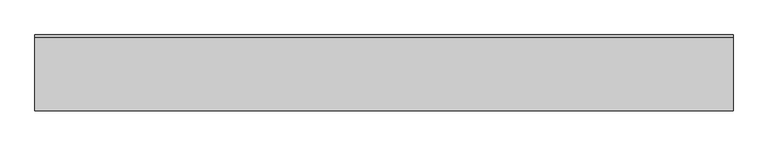
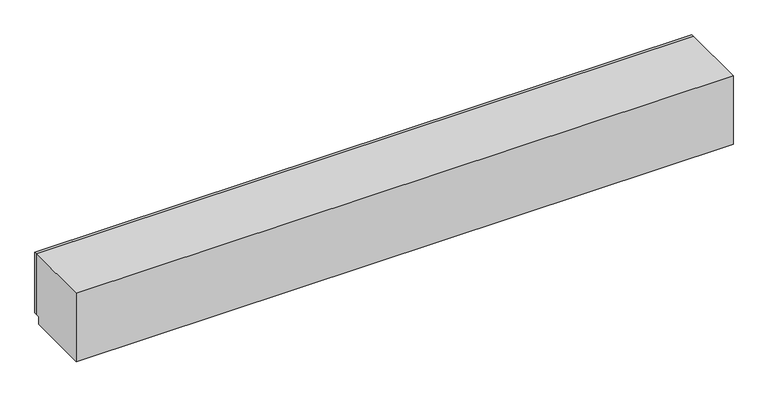
"""IFC4 building model written with IfcOpenShell, lengths in millimetres: furniture geometry, OD_CW_Base Cabinet : OD_CW_Base Cabinet."""

from ifc_helpers import new_model, si_unit, frame, origin, place, context, project, spatial, polyline, outline, extrude, source, transform, mapped, element, save


def furniture_861fb723(model_context):
    return source(origin(), model_context, "Body", "SweptSolid", [
        extrude(outline(polyline([(18.7377049, 228.6), (18.7377049, 254.0), (7982.4770576, 254.0), (7982.4770576, 228.6), (18.7377049, 228.6)])), frame((0.0, 0.0, 101.6), z_axis=(0.0, 0.0, 1.0), x_axis=(1.0, 0.0, 0.0)), (0.0, 0.0, 1.0), 774.7),
        extrude(outline(polyline([(228.6, 876.3), (228.6, 101.6), (177.8, 101.6), (177.8, 0.0), (-609.6, 0.0), (-609.6, 876.3), (228.6, 876.3)])), frame((18.7377049, 0.0, 0.0), z_axis=(1.0, 0.0, 0.0), x_axis=(0.0, 1.0, 0.0)), (0.0, 0.0, 1.0), 7963.7393527),
    ])


if __name__ == "__main__":
    model = new_model("IFC4")
    model_context = context("Model", 3, world=origin())
    ifc_project = project(units=[si_unit("LENGTHUNIT", "METRE", prefix="MILLI")], contexts=[model_context])
    site = spatial("IfcSite", under=ifc_project)
    building = spatial("IfcBuilding", under=site)
    placement = place(None, origin())
    furniture_shape = furniture_861fb723(model_context)
    element("IfcFurniture", 1, ObjectType="OD_CW_Base Cabinet : OD_CW_Base Cabinet", at=placement, inside=building, context=model_context, shape_type="MappedRepresentation", body=[
        mapped(furniture_shape, transform((0.0, 0.0, 0.0), x_axis=(1.0, 0.0, 0.0), y_axis=(0.0, 1.0, 0.0), z_axis=(0.0, 0.0, 1.0))),
    ])
    save(model, "model.ifc")

# Revit data of these elements
# Type "OD_CW_Base Cabinet : OD_CW_Base Cabinet"
#   OD_CW_Width [instance default] = 2' - 10"
#   OD_CW_Length [instance default] = 8' - 0"
#   OD_CW_Height [instance default] = 2' - 3"
#   Depth = 2' - 0"
#   Height = 3' - 0"
#   Width = 4' - 0"
#   OD_CW_Material_Front Panel [instance default] = none
#   OD_CW_Material_Body [instance default] = none
# Element 1 (IfcFurniture, "OD_CW_Base Cabinet : OD_CW_Base Cabinet")
#   OD_CW_Length = 26' - 1.53305"
#   OD_CW_Height = 2' - 10 1/2"
#   Materials on its faces: "CASEWORK"
# Materials
#   "CASEWORK": class "Generic", colour RGB 181 181 181, transparency 0, Cost = 0
